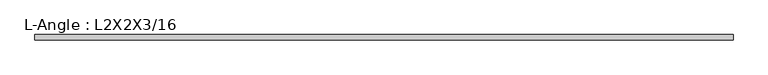
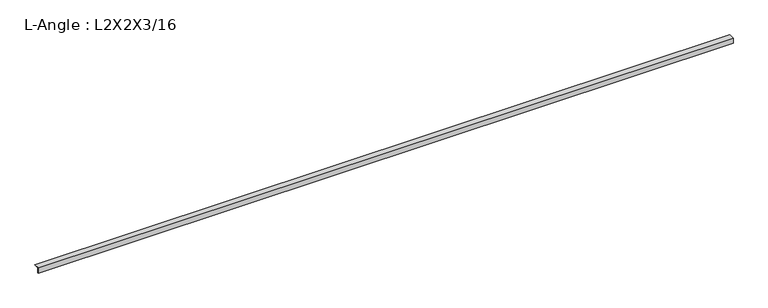
"""IFC4 building model written with IfcOpenShell, lengths in millimetres: beam geometry, L-Angle : L2X2X3/16."""

from ifc_helpers import new_model, si_unit, point, frame, frame_2d, origin, place, context, project, spatial, polyline, circle_curve, trimmed, segment, composite_curve, outline, extrude, source, transform, mapped, element, save


def l_angle_l2x2x3_16_5de402f4(model_context):
    return source(origin(), model_context, "Body", "SweptSolid", [
        extrude(outline(composite_curve([segment(polyline([(-14.2494, 14.2494), (36.5506, 14.2494)]), True, "CONTINUOUS"), segment(trimmed(circle_curve(frame_2d((31.7881, 14.2494)), 4.7625), [point((36.5506, 14.2494))], [point((31.7881, 9.4869))], False, "CARTESIAN"), True, "CONTINUOUS"), segment(polyline([(31.7881, 9.4869), (-4.7244, 9.4869)]), True, "CONTINUOUS"), segment(trimmed(circle_curve(frame_2d((-4.7244, 4.7244)), 4.7625), [point((-4.7244, 9.4869))], [point((-9.4869, 4.7244))], True, "CARTESIAN"), True, "CONTINUOUS"), segment(polyline([(-9.4869, 4.7244), (-9.4869, -31.7881)]), True, "CONTINUOUS"), segment(trimmed(circle_curve(frame_2d((-14.2494, -31.7881)), 4.7625), [point((-9.4869, -31.7881))], [point((-14.2494, -36.5506))], False, "CARTESIAN"), True, "CONTINUOUS"), segment(polyline([(-14.2494, -36.5506), (-14.2494, 14.2494)]), True, "CONTINUOUS")], self_intersect=False)), frame((-3252.7874994, 0.0, 0.0), z_axis=(1.0, 0.0, 0.0), x_axis=(0.0, 1.0, 0.0)), (0.0, 0.0, 1.0), 6346.8249994),
    ])


if __name__ == "__main__":
    model = new_model("IFC4")
    model_context = context("Model", 3, world=origin())
    ifc_project = project(units=[si_unit("LENGTHUNIT", "METRE", prefix="MILLI")], contexts=[model_context])
    site = spatial("IfcSite", under=ifc_project)
    building = spatial("IfcBuilding", under=site)
    placement = place(None, origin())
    l_angle_l2x2x3_16_shape = l_angle_l2x2x3_16_5de402f4(model_context)
    element("IfcBeam", 1, ObjectType="L-Angle : L2X2X3/16", at=placement, inside=building, context=model_context, shape_type="MappedRepresentation", body=[
        mapped(l_angle_l2x2x3_16_shape, transform((0.0, 0.0, 0.0), x_axis=(1.0, 0.0, 0.0), y_axis=(0.0, 1.0, 0.0), z_axis=(0.0, 0.0, 1.0))),
    ])
    save(model, "model.ifc")

# Revit data of these elements
# Type "L-Angle : L2X2X3/16"
#   Assembly Code = "B10"
#   k = 0' - 0 7/16"
#   W = 2.44
#   Start Extension Calculation [instance default] = 10' - 0"
#   Start Extension [instance default] = -0' - 0 1/2"
#   End Extension Calculation [instance default] = 10' - 0"
#   End Extension [instance default] = -0' - 0 1/2"
#   Length [instance default] = 5' - 0"
#   b = 0' - 2"
#   d = 0' - 2"
#   t = 0' - 0 3/16"
#   x = 0' - 0.561"
#   y = 0' - 0.561"
#   A = 0.00496528 SF
#   Structural Material [instance default] = Metal - Steel - ASTM A36
# Element 1 (IfcBeam, "L-Angle : L2X2X3/16")
#   Structural Material = STRUCTURAL STEEL - SEE STRUCT. DWGS
#   Materials on its faces: "STRUCTURAL STEEL - SEE STRUCT. DWGS"
# Materials
#   "Metal - Steel - ASTM A36": class "Metal", colour RGB 199 199 199, transparency 0
#   "STRUCTURAL STEEL - SEE STRUCT. DWGS": class "Metal", colour RGB 137 146 153, transparency 0, Description = "Steel, mill finish", Cost = 0
